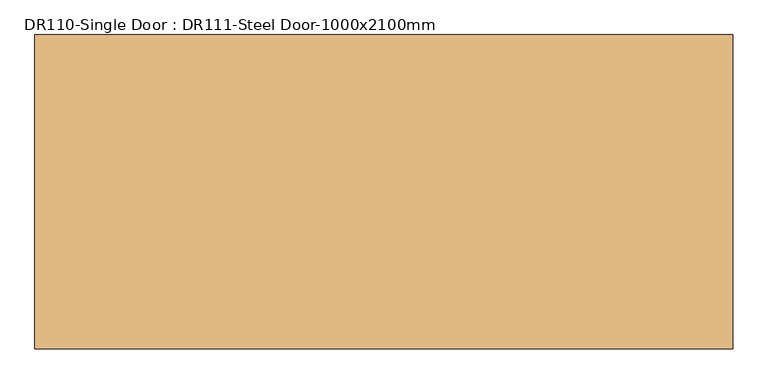
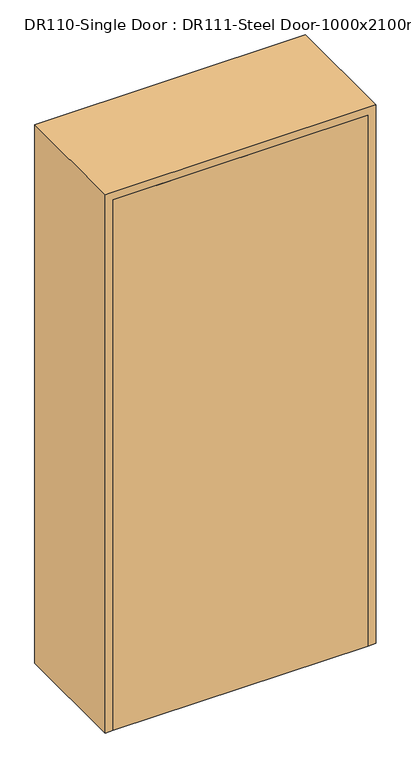
"""IFC4 building model written with IfcOpenShell, lengths in millimetres: door geometry, DR110-Single Door : DR111-Steel Door-1000x2100mm."""

from ifc_helpers import new_model, si_unit, origin, origin_with_axes, place, context, project, spatial, polyline, outline, extrude, faceted_brep, source, transform, mapped, element, save


def dr110_single_door_dr111_steel_door_1000x2100mm_3adf1b50(model_context):
    return source(origin(), model_context, "Body", "SolidModel", [
        extrude(outline(polyline([(470.0, -225.0), (-470.0, -225.0), (-470.0, -190.0), (470.0, -190.0), (470.0, -225.0)])), origin_with_axes(), (0.0, 0.0, 1.0), 2070.0),
        faceted_brep([(470.0, -225.0, 0.0), (470.0, -190.0, 0.0), (450.0, -190.0, 0.0), (450.0, 190.0, 0.0), (470.0, 190.0, 0.0), (470.0, 225.0, 0.0), (500.0, 225.0, 0.0), (500.0, -225.0, 0.0), (500.0, -225.0, 2100.0), (-500.0, -225.0, 2100.0), (-500.0, -225.0, 0.0), (-470.0, -225.0, 0.0), (-470.0, -225.0, 2070.0), (470.0, -225.0, 2070.0), (500.0, 225.0, 2100.0), (470.0, 225.0, 2070.0), (-470.0, 225.0, 2070.0), (-470.0, 225.0, 0.0), (-500.0, 225.0, 0.0), (-500.0, 225.0, 2100.0), (470.0, 190.0, 2070.0), (450.0, 190.0, 2050.0), (-450.0, 190.0, 2050.0), (-450.0, 190.0, 0.0), (-470.0, 190.0, 0.0), (-470.0, 190.0, 2070.0), (450.0, -190.0, 2050.0), (470.0, -190.0, 2070.0), (-470.0, -190.0, 2070.0), (-470.0, -190.0, 0.0), (-450.0, -190.0, 0.0), (-450.0, -190.0, 2050.0)], [[[0, 1, 2, 3, 4, 5, 6, 7]], [[7, 8, 9, 10, 11, 12, 13, 0]], [[6, 14, 8, 7]], [[5, 15, 16, 17, 18, 19, 14, 6]], [[4, 20, 15, 5]], [[3, 21, 22, 23, 24, 25, 20, 4]], [[2, 26, 21, 3]], [[1, 27, 28, 29, 30, 31, 26, 2]], [[0, 13, 27, 1]], [[12, 11, 29, 28]], [[11, 10, 18, 17, 24, 23, 30, 29]], [[19, 18, 10, 9]], [[25, 24, 17, 16]], [[31, 30, 23, 22]], [[14, 19, 9, 8]], [[20, 25, 16, 15]], [[26, 31, 22, 21]], [[13, 12, 28, 27]]]),
    ])


if __name__ == "__main__":
    model = new_model("IFC4")
    model_context = context("Model", 3, world=origin())
    ifc_project = project(units=[si_unit("LENGTHUNIT", "METRE", prefix="MILLI")], contexts=[model_context])
    site = spatial("IfcSite", under=ifc_project)
    building = spatial("IfcBuilding", under=site)
    placement = place(None, origin())
    dr110_single_door_dr111_steel_door_1000x2100mm_shape = dr110_single_door_dr111_steel_door_1000x2100mm_3adf1b50(model_context)
    element("IfcDoor", 1, ObjectType="DR110-Single Door : DR111-Steel Door-1000x2100mm", at=placement, inside=building, context=model_context, shape_type="MappedRepresentation", body=[
        mapped(dr110_single_door_dr111_steel_door_1000x2100mm_shape, transform((0.0, 0.0, 0.0), x_axis=(1.0, 0.0, 0.0), y_axis=(0.0, 1.0, 0.0), z_axis=(0.0, 0.0, 1.0))),
    ])
    save(model, "model.ifc")

# Revit data of these elements
# Type "DR110-Single Door : DR111-Steel Door-1000x2100mm"
#   Type Mark = "SD"
#   Analytic Construction = "<None>"
#   프레임 투영 외부. = 25 mm
#   프레임 투영 내부. = 25 mm
#   프레임 폭 = 75 mm
#   Height = 2100 mm
#   Width = 1000 mm
#   Define Thermal Properties by = 1
#   문 패널 = SD1 문 패널
#   문 프레임 = A04AQ098-00002_Steel Door_non FP_single
#   Function = (empty or 0)
#   Wall Closure = (empty or 0)
# Element 1 (IfcDoor, "DR110-Single Door : DR111-Steel Door-1000x2100mm")
#   Materials on its faces: "A04AQ098-00002_Steel Door_non FP_single", "SD1 문 패널"
# Materials
#   "SD1 문 패널": class "금속", colour RGB 247 247 247, transparency 0, Description = "STEEL DOOR (1000Wx2100H)"
#   "A04AQ098-00002_Steel Door_non FP_single": class "금속", colour RGB 247 247 247, transparency 0, Description = "Steel Door", W00) Work Master Code = "A04AQ098-00002", W01) Work Master_Lv1 = "Finishing Work", W02) Work Master_Lv2 = "Door & Window Work", W03) Work Master_Spec.1 = "Steel Door w/ Steel Frame", W04) Work Master_Spec.2 = "Fire Protective Rating: N/A, Single Door", W05) Work Master_Spec.3 = "w/ Hardware & Accessories", Cost = 0
